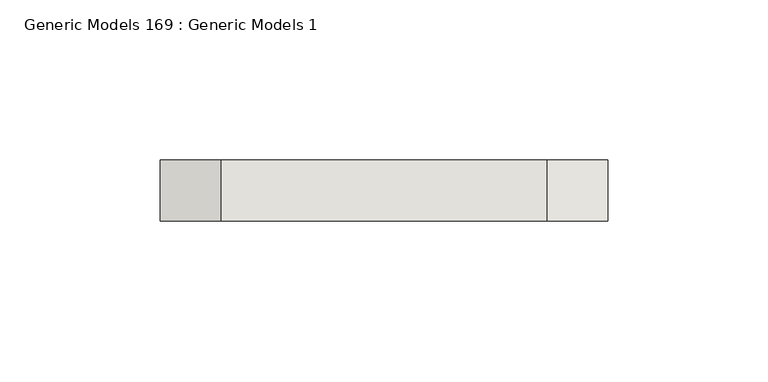
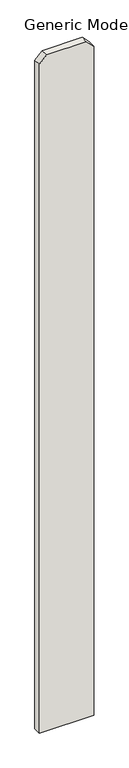
"""IFC4 building model written with IfcOpenShell, lengths in millimetres: wall geometry, Generic Models 169 : Generic Models 1."""

from ifc_helpers import new_model, si_unit, frame, origin, place, context, project, spatial, polyline, outline, extrude, source, transform, mapped, element, save


def generic_models_169_generic_models_1_d5021c3c(model_context):
    return source(origin(), model_context, "Body", "SweptSolid", [
        extrude(outline(polyline([(76.2, 324737.4125), (1885.95, 324737.4125), (1905.0, 324718.3625), (1905.0, 324616.7625), (1885.95, 324597.7125), (76.2, 324597.7125), (76.2, 324737.4125)])), frame((0.0, 547.6875, 0.0), z_axis=(0.0, 1.0, 0.0), x_axis=(0.0, 0.0, 1.0)), (0.0, 0.0, 1.0), 19.05),
    ])


if __name__ == "__main__":
    model = new_model("IFC4")
    model_context = context("Model", 3, world=origin())
    ifc_project = project(units=[si_unit("LENGTHUNIT", "METRE", prefix="MILLI")], contexts=[model_context])
    site = spatial("IfcSite", under=ifc_project)
    building = spatial("IfcBuilding", under=site)
    placement = place(None, origin())
    generic_models_169_generic_models_1_shape = generic_models_169_generic_models_1_d5021c3c(model_context)
    element("IfcWall", 1, ObjectType="Generic Models 169 : Generic Models 1", at=placement, inside=building, context=model_context, shape_type="MappedRepresentation", body=[
        mapped(generic_models_169_generic_models_1_shape, transform((0.0, 0.0, 0.0), x_axis=(1.0, 0.0, 0.0), y_axis=(0.0, 1.0, 0.0), z_axis=(0.0, 0.0, 1.0))),
    ])
    save(model, "model.ifc")

# Revit data of these elements
# Element 1 (IfcWall, "Generic Models 169 : Generic Models 1")
#   Materials on its faces: "VERTICAL 1X6 CEDAR PLANKS W/ CLEAR WOOD SEALER"
# Materials
#   "VERTICAL 1X6 CEDAR PLANKS W/ CLEAR WOOD SEALER": class "Wood", colour RGB 234 198 147, transparency 0, Description = "Pinus Echinata", Cost = 0
